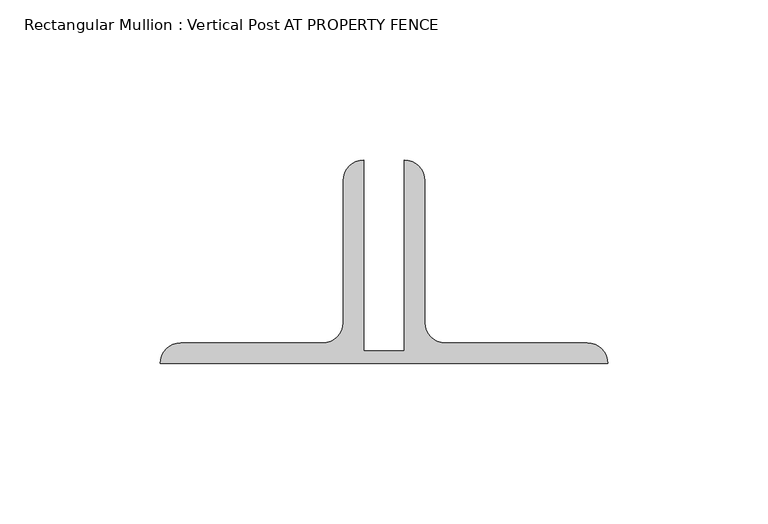
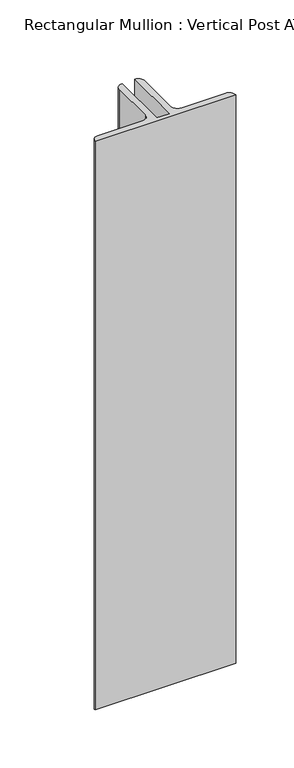
"""IFC4 building model written with IfcOpenShell, lengths in millimetres: member geometry, Rectangular Mullion : Vertical Post AT PROPERTY FENCE."""

from ifc_helpers import new_model, si_unit, point, frame, frame_2d, origin, place, context, project, spatial, polyline, circle_curve, trimmed, segment, composite_curve, outline, extrude, source, transform, mapped, element, save


def rectangular_mullion_vertical_post_at_property_fence_a50c0036(model_context):
    return source(origin(), model_context, "Body", "SweptSolid", [
        extrude(outline(composite_curve([segment(polyline([(-6.35, 22.9145205), (6.35, 22.9145205), (6.35, 82.55)]), True, "CONTINUOUS"), segment(trimmed(circle_curve(frame_2d((6.35, 76.2)), 6.35), [point((6.35, 82.55))], [point((12.7, 76.2))], False, "CARTESIAN"), True, "CONTINUOUS"), segment(polyline([(12.7, 76.2), (12.7, 31.75)]), True, "CONTINUOUS"), segment(trimmed(circle_curve(frame_2d((19.05, 31.75)), 6.35), [point((12.7, 31.75))], [point((19.05, 25.4))], True, "CARTESIAN"), True, "CONTINUOUS"), segment(polyline([(19.05, 25.4), (63.5, 25.4)]), True, "CONTINUOUS"), segment(trimmed(circle_curve(frame_2d((63.5, 19.05)), 6.35), [point((63.5, 25.4))], [point((69.85, 19.05))], False, "CARTESIAN"), True, "CONTINUOUS"), segment(polyline([(69.85, 19.05), (-69.85, 19.05)]), True, "CONTINUOUS"), segment(trimmed(circle_curve(frame_2d((-63.5, 19.05)), 6.35), [point((-69.85, 19.05))], [point((-63.5, 25.4))], False, "CARTESIAN"), True, "CONTINUOUS"), segment(polyline([(-63.5, 25.4), (-19.05, 25.4)]), True, "CONTINUOUS"), segment(trimmed(circle_curve(frame_2d((-19.05, 31.75)), 6.35), [point((-19.05, 25.4))], [point((-12.7, 31.75))], True, "CARTESIAN"), True, "CONTINUOUS"), segment(polyline([(-12.7, 31.75), (-12.7, 76.2)]), True, "CONTINUOUS"), segment(trimmed(circle_curve(frame_2d((-6.35, 76.2)), 6.35), [point((-12.7, 76.2))], [point((-6.35, 82.55))], False, "CARTESIAN"), True, "CONTINUOUS"), segment(polyline([(-6.35, 82.55), (-6.35, 22.9145205)]), True, "CONTINUOUS")], self_intersect=False)), frame((0.0, 0.0, -596.9), z_axis=(0.0, 0.0, 1.0), x_axis=(1.0, 0.0, 0.0)), (0.0, 0.0, 1.0), 596.9),
    ])


if __name__ == "__main__":
    model = new_model("IFC4")
    model_context = context("Model", 3, world=origin())
    ifc_project = project(units=[si_unit("LENGTHUNIT", "METRE", prefix="MILLI")], contexts=[model_context])
    site = spatial("IfcSite", under=ifc_project)
    building = spatial("IfcBuilding", under=site)
    placement = place(None, origin())
    rectangular_mullion_vertical_post_at_property_fence_shape = rectangular_mullion_vertical_post_at_property_fence_a50c0036(model_context)
    element("IfcMember", 1, ObjectType="Rectangular Mullion : Vertical Post AT PROPERTY FENCE", at=placement, inside=building, context=model_context, shape_type="MappedRepresentation", body=[
        mapped(rectangular_mullion_vertical_post_at_property_fence_shape, transform((0.0, 0.0, 0.0), x_axis=(1.0, 0.0, 0.0), y_axis=(0.0, 1.0, 0.0), z_axis=(0.0, 0.0, 1.0))),
    ])
    save(model, "model.ifc")

# Revit data of these elements
# Type "Rectangular Mullion : Vertical Post AT PROPERTY FENCE"
#   built-in parameter 1007351 = -0.0625 (stored number, unit not read)
#   built-in parameter 1007322 = 0.0126789 (stored number, unit not read)
#   built-in parameter 1007321 = 0.229167 (stored number, unit not read)
#   built-in parameter 1007320 = 0.229167 (stored number, unit not read)
# Element 1 (IfcMember, "Rectangular Mullion : Vertical Post AT PROPERTY FENCE")
#   Materials on its faces: "MAIN FENCE POST: (2) BACK/BACK GALVANIZED ANGLES (2) L2 1/2 X 2 1/2 X 1/4\") ANCHORED TO 8\"W X 42\" DEEP CONCRETE FOOTING(1)"
# Materials
#   "MAIN FENCE POST: (2) BACK/BACK GALVANIZED ANGLES (2) L2 1/2 X 2 1/2 X 1/4\") ANCHORED TO 8\"W X 42\" DEEP CONCRETE FOOTING(1)": class "Unassigned", colour RGB 211 211 211, transparency 0, Cost = 0
